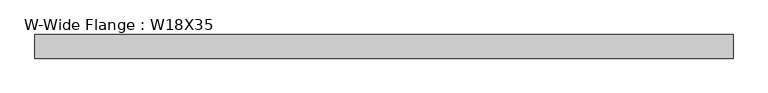
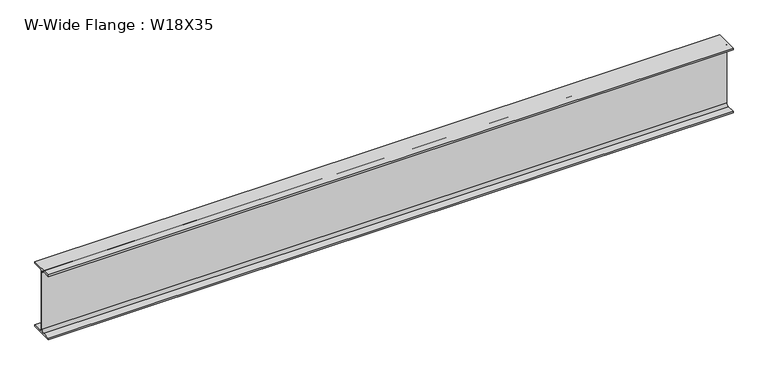
"""IFC4 building model written with IfcOpenShell, lengths in millimetres: beam geometry, W-Wide Flange : W18X35."""

from ifc_helpers import new_model, si_unit, point, frame, frame_2d, origin, place, context, project, spatial, polyline, circle_curve, trimmed, segment, composite_curve, outline, extrude, source, transform, mapped, element, save


def w_wide_flange_w18x35_ad683e90(model_context):
    return source(origin(), model_context, "Body", "SweptSolid", [
        extrude(outline(composite_curve([segment(polyline([(76.2, -213.995), (76.2, -224.79), (-76.2, -224.79), (-76.2, -213.995), (-21.59, -213.995)]), True, "CONTINUOUS"), segment(trimmed(circle_curve(frame_2d((-21.59, -196.215)), 17.78), [point((-21.59, -213.995))], [point((-3.81, -196.215))], True, "CARTESIAN"), True, "CONTINUOUS"), segment(polyline([(-3.81, -196.215), (-3.81, 196.215)]), True, "CONTINUOUS"), segment(trimmed(circle_curve(frame_2d((-21.59, 196.215)), 17.78), [point((-3.81, 196.215))], [point((-21.59, 213.995))], True, "CARTESIAN"), True, "CONTINUOUS"), segment(polyline([(-21.59, 213.995), (-76.2, 213.995), (-76.2, 224.79), (76.2, 224.79), (76.2, 213.995), (21.59, 213.995)]), True, "CONTINUOUS"), segment(trimmed(circle_curve(frame_2d((21.59, 196.215)), 17.78), [point((21.59, 213.995))], [point((3.81, 196.215))], True, "CARTESIAN"), True, "CONTINUOUS"), segment(polyline([(3.81, 196.215), (3.81, -196.215)]), True, "CONTINUOUS"), segment(trimmed(circle_curve(frame_2d((21.59, -196.215)), 17.78), [point((3.81, -196.215))], [point((21.59, -213.995))], True, "CARTESIAN"), True, "CONTINUOUS"), segment(polyline([(21.59, -213.995), (76.2, -213.995)]), True, "CONTINUOUS")], self_intersect=False)), frame((-2247.9, 0.0, 0.0), z_axis=(1.0, 0.0, 0.0), x_axis=(0.0, 1.0, 0.0)), (0.0, 0.0, 1.0), 4495.8),
    ])


if __name__ == "__main__":
    model = new_model("IFC4")
    model_context = context("Model", 3, world=origin())
    ifc_project = project(units=[si_unit("LENGTHUNIT", "METRE", prefix="MILLI")], contexts=[model_context])
    site = spatial("IfcSite", under=ifc_project)
    building = spatial("IfcBuilding", under=site)
    placement = place(None, origin())
    w_wide_flange_w18x35_shape = w_wide_flange_w18x35_ad683e90(model_context)
    element("IfcBeam", 1, ObjectType="W-Wide Flange : W18X35", at=placement, inside=building, context=model_context, shape_type="MappedRepresentation", body=[
        mapped(w_wide_flange_w18x35_shape, transform((0.0, 0.0, 0.0), x_axis=(1.0, 0.0, 0.0), y_axis=(0.0, 1.0, 0.0), z_axis=(0.0, 0.0, 1.0))),
    ])
    save(model, "model.ifc")

# Revit data of these elements
# Type "W-Wide Flange : W18X35"
#   Assembly Code = "B10"
#   W = 35
#   Length [instance default] = 5' - 0"
#   bf = 0' - 6"
#   d = 1' - 5.7"
#   k = 0' - 1 1/8"
#   k2 = 0' - 0.7"
#   tf = 0' - 0.425"
#   tw = 0' - 0.3"
#   A = 0.0715278 SF
#   Structural Material [instance default] = Steel ASTM A992
# Element 1 (IfcBeam, "W-Wide Flange : W18X35")
#   Structural Material = Steel ASTM A36
#   Materials on its faces: "Steel ASTM A36"
# Materials
#   "Steel ASTM A992": class "Metal", colour RGB 199 199 199, transparency 0, Description = "Structural steel 50ksi", Cost = 0
#   "Steel ASTM A36": class "Metal", colour RGB 199 199 199, transparency 0, Description = "Structural steel, ASTM A36 Grade B, mill finish", Cost = 0
